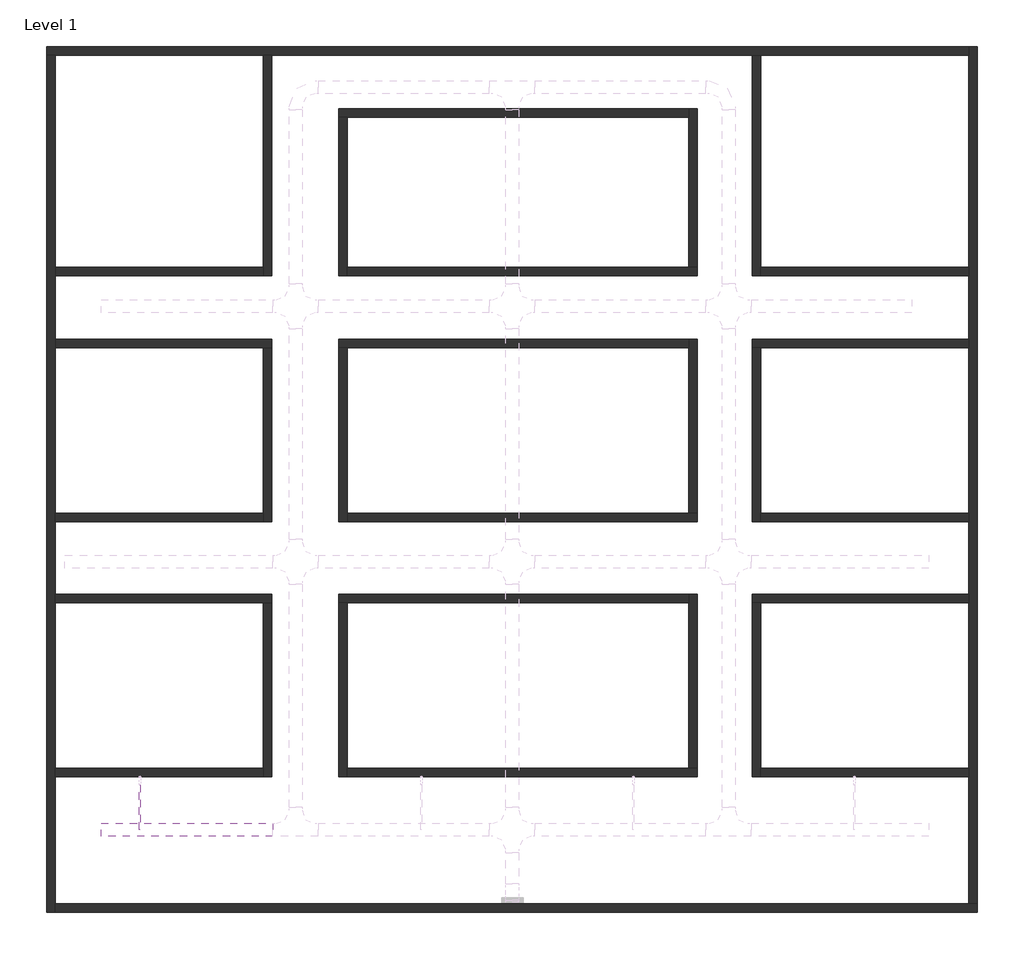
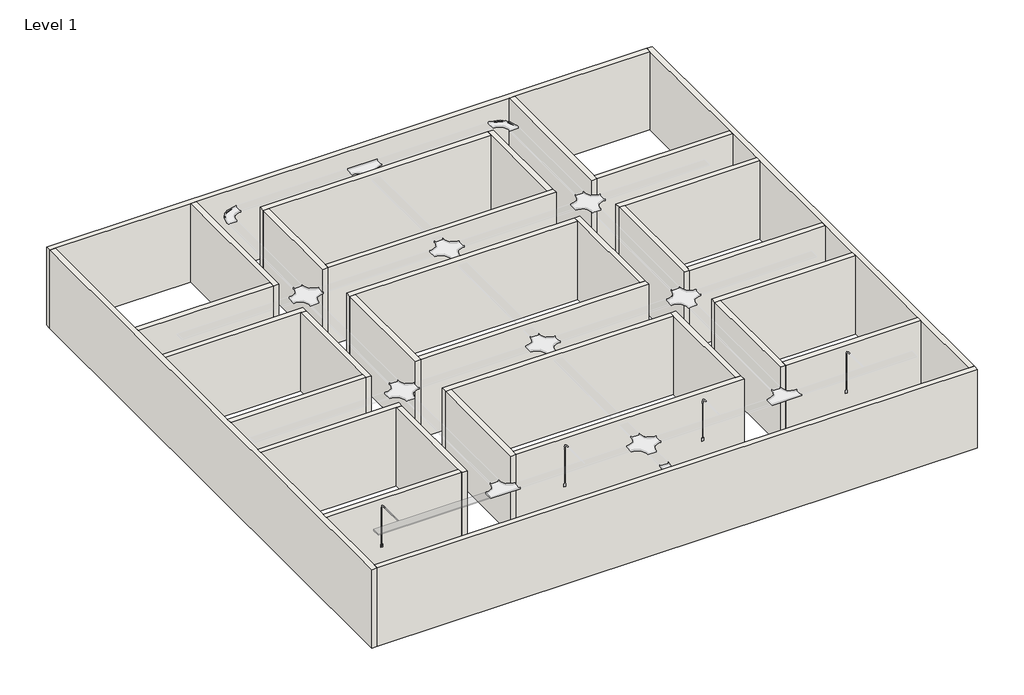
# One storey, part 1 of 2: 32 walls, 3 cable carrier segments, 1 proxy.
"""IFC4 building model written with IfcOpenShell, lengths in millimetres."""

import ifcopenshell
import ifcopenshell.guid

model = None  # the IFC model being written
_history = None  # IfcOwnerHistory: only IFC2X3 demands one
_inside = {}  # id of a spatial element -> (the spatial element, [elements in it])
_under = {}  # id of a project, library or spatial element -> (it, [spatial elements below it])
_declared = {}  # id of a project -> (the project, [libraries it declares])
_typed = {}  # id of a type object -> (the type object, [elements of that type])
_made_of = {}  # id of a material, layer set ... -> (it, [elements and type objects made of it])


def new_model(schema):
    """Start an empty IFC model of exactly this schema.

    Asked for "IFC4X3", IfcOpenShell would pick the latest addendum, in which some entities
    have other attributes; the version numbers below select the first issue.
    IFC2X3 requires an IfcOwnerHistory on every rooted entity: one is made here for all.
    """
    global model, _history
    if schema == "IFC4X3":
        model = ifcopenshell.file(schema_version=(4, 3, 0, 0))
    else:
        model = ifcopenshell.file(schema=schema)
    _inside.clear()
    _under.clear()
    _declared.clear()
    _typed.clear()
    _made_of.clear()
    _history = None
    if model.schema == "IFC2X3":
        org = make("IfcOrganization", Name="unknown")
        user = make(
            "IfcPersonAndOrganization",
            ThePerson=make("IfcPerson", FamilyName="unknown"),
            TheOrganization=org,
        )
        app = make(
            "IfcApplication",
            ApplicationDeveloper=org,
            Version="unknown",
            ApplicationFullName="unknown",
            ApplicationIdentifier="unknown",
        )
        _history = make(
            "IfcOwnerHistory",
            OwningUser=user,
            OwningApplication=app,
            ChangeAction="ADDED",
            CreationDate=0,
        )
    return model


def make(cls, **values):
    """One entity of the class cls with the attributes given. An attribute that is None is left unset."""
    return model.create_entity(
        cls, **{name: value for name, value in values.items() if value is not None}
    )


def rooted(cls, **values):
    """An entity with a GlobalId (a new one), such as an element, a storey or a relation."""
    return make(cls, GlobalId=ifcopenshell.guid.new(), OwnerHistory=_history, **values)


def si_unit(unit_type, name, prefix=None):
    """IfcSIUnit, for example si_unit("LENGTHUNIT", "METRE", prefix="MILLI")."""
    return make("IfcSIUnit", UnitType=unit_type, Prefix=prefix, Name=name)


def assignment(units):
    """IfcUnitAssignment: the units of a project."""
    return None if units is None else make("IfcUnitAssignment", Units=units)


def point(xyz):
    """IfcCartesianPoint."""
    return None if xyz is None else make("IfcCartesianPoint", Coordinates=xyz)


def direction(xyz):
    """IfcDirection."""
    return None if xyz is None else make("IfcDirection", DirectionRatios=xyz)


def frame(location, z_axis=None, x_axis=None):
    """IfcAxis2Placement3D, a coordinate frame: its origin and axes. An axis left out is left unset."""
    return make(
        "IfcAxis2Placement3D",
        Location=point(location),
        Axis=direction(z_axis),
        RefDirection=direction(x_axis),
    )


def frame_2d(location, x_axis=None):
    """IfcAxis2Placement2D, a coordinate frame in the plane: its origin and x axis."""
    return make(
        "IfcAxis2Placement2D", Location=point(location), RefDirection=direction(x_axis)
    )


def origin():
    """The frame at (0, 0, 0) with its axes left unset."""
    return frame((0.0, 0.0, 0.0))


def origin_with_axes():
    """The frame at (0, 0, 0) with the z axis (0, 0, 1) and the x axis (1, 0, 0) written out."""
    return frame((0.0, 0.0, 0.0), z_axis=(0.0, 0.0, 1.0), x_axis=(1.0, 0.0, 0.0))


def place(relative_to, where):
    """IfcLocalPlacement: puts the frame where relative to a parent placement (None: the world)."""
    return make(
        "IfcLocalPlacement", PlacementRelTo=relative_to, RelativePlacement=where
    )


def context(
    kind, dimensions, precision=None, world=None, true_north=None, identifier=None
):
    """IfcGeometricRepresentationContext, for example the 3D "Model" context."""
    return make(
        "IfcGeometricRepresentationContext",
        ContextIdentifier=identifier,
        ContextType=kind,
        CoordinateSpaceDimension=dimensions,
        Precision=precision,
        WorldCoordinateSystem=world,
        TrueNorth=true_north,
    )


def project(units=None, contexts=None):
    """IfcProject with its units and contexts."""
    return rooted(
        "IfcProject",
        Name="project",
        RepresentationContexts=contexts,
        UnitsInContext=assignment(units),
    )


def spatial(cls, under=None, at=None, **own):
    """A site, building, storey or space (cls), placed at a placement, below another one or the project."""
    s = rooted(cls, ObjectPlacement=at, **own)
    if under is not None:
        _under.setdefault(under.id(), (under, []))[1].append(s)
    return s


def polyline(points):
    """IfcPolyline through the points."""
    return make("IfcPolyline", Points=[point(p) for p in points])


def circle_curve(where, radius):
    """IfcCircle in the frame where."""
    return make("IfcCircle", Position=where, Radius=radius)


def trimmed(basis, trim1, trim2, sense, master):
    """IfcTrimmedCurve: the piece of a basis curve between two trims."""
    return make(
        "IfcTrimmedCurve",
        BasisCurve=basis,
        Trim1=trim1,
        Trim2=trim2,
        SenseAgreement=sense,
        MasterRepresentation=master,
    )


def segment(curve, same_sense, transition):
    """IfcCompositeCurveSegment."""
    return make(
        "IfcCompositeCurveSegment",
        Transition=transition,
        SameSense=same_sense,
        ParentCurve=curve,
    )


def composite_curve(segments, self_intersect=None):
    """IfcCompositeCurve: segments joined end to end."""
    return make("IfcCompositeCurve", Segments=segments, SelfIntersect=self_intersect)


def outline(outer, holes=None, kind="AREA"):
    """IfcArbitraryClosedProfileDef: a profile drawn as a closed curve; with holes, ...WithVoids."""
    if holes is None:
        return make("IfcArbitraryClosedProfileDef", ProfileType=kind, OuterCurve=outer)
    return make(
        "IfcArbitraryProfileDefWithVoids",
        ProfileType=kind,
        OuterCurve=outer,
        InnerCurves=holes,
    )


def extrude(swept, where, along, depth):
    """IfcExtrudedAreaSolid: the profile swept, set in the frame where, extruded along a direction by depth."""
    return make(
        "IfcExtrudedAreaSolid",
        SweptArea=swept,
        Position=where,
        ExtrudedDirection=direction(along),
        Depth=depth,
    )


def faces_of(points, faces, orient=None, outer=None):
    """IfcFace entities. A face is a list of loops; a loop is a list of indices into points, from 0.

    orient and outer hold one flag for each loop. By default every Orientation is true, the
    first loop of a face is its IfcFaceOuterBound and the others are IfcFaceBound.
    """
    made = []
    for i, loops in enumerate(faces):
        bounds = []
        for j, loop in enumerate(loops):
            is_outer = j == 0 if outer is None else outer[i][j]
            bounds.append(
                make(
                    "IfcFaceOuterBound" if is_outer else "IfcFaceBound",
                    Bound=make("IfcPolyLoop", Polygon=[points[k] for k in loop]),
                    Orientation=True if orient is None else orient[i][j],
                )
            )
        made.append(make("IfcFace", Bounds=bounds))
    return made


def faceted_brep(points, faces, orient=None, outer=None, voids=None):
    """IfcFacetedBrep: a solid bounded by flat faces; with voids (closed shells), ...WithVoids."""
    shared = [point(p) for p in points]
    hull = make("IfcClosedShell", CfsFaces=faces_of(shared, faces, orient, outer))
    if voids is None:
        return make("IfcFacetedBrep", Outer=hull)
    return make(
        "IfcFacetedBrepWithVoids",
        Outer=hull,
        Voids=[
            make(cls, CfsFaces=faces_of(shared, fs, o, b)) for cls, fs, o, b in voids
        ],
    )


def shape(context_of_items, identifier, shape_type, items):
    """IfcShapeRepresentation: the items that make up one representation, for example the "Body"."""
    return make(
        "IfcShapeRepresentation",
        ContextOfItems=context_of_items,
        RepresentationIdentifier=identifier,
        RepresentationType=shape_type,
        Items=items,
    )


def source(mapping_origin, context_of_items, identifier, shape_type, items):
    """IfcRepresentationMap: a shape defined once, which mapped items show again and again."""
    return make(
        "IfcRepresentationMap",
        MappingOrigin=mapping_origin,
        MappedRepresentation=shape(context_of_items, identifier, shape_type, items),
    )


def transform(
    local_origin,
    x_axis=None,
    y_axis=None,
    z_axis=None,
    scale=None,
    scale2=None,
    scale3=None,
    uniform=True,
):
    """IfcCartesianTransformationOperator3D, or its non-uniform kind. x_axis, y_axis, z_axis: its Axis1, 2, 3."""
    if uniform:
        return make(
            "IfcCartesianTransformationOperator3D",
            Axis1=direction(x_axis),
            Axis2=direction(y_axis),
            LocalOrigin=point(local_origin),
            Scale=scale,
            Axis3=direction(z_axis),
        )
    return make(
        "IfcCartesianTransformationOperator3DnonUniform",
        Axis1=direction(x_axis),
        Axis2=direction(y_axis),
        LocalOrigin=point(local_origin),
        Scale=scale,
        Axis3=direction(z_axis),
        Scale2=scale2,
        Scale3=scale3,
    )


def mapped(mapping_source, mapping_target):
    """IfcMappedItem: shows the shape of a source again, moved by a transform."""
    return make(
        "IfcMappedItem", MappingSource=mapping_source, MappingTarget=mapping_target
    )


def made_of(thing, what):
    """Note that an element or type object is made of a material, layer set ...; save() writes the relation."""
    if what is not None:
        _made_of.setdefault(what.id(), (what, []))[1].append(thing)
    return thing


def element(
    cls,
    number,
    at=None,
    inside=None,
    cuts=None,
    type_object=None,
    material=None,
    context=None,
    identifier="Body",
    shape_type=None,
    held_by="IfcProductDefinitionShape",
    body=None,
    shapes=None,
    **own,
):
    """One element of the class cls, such as IfcWall. Its Tag is "e" and its number.

    at: its placement. inside: the storey or other place that contains it. cuts: it is an
    opening in that element (IfcRelVoidsElement). A single representation is given by context,
    identifier, shape_type and body (its items); several are given by shapes. held_by: the class
    of the entity that holds the representations. save() writes the other relations.
    """
    e = rooted(cls, Tag="e%d" % number, ObjectPlacement=at, **own)
    if body is not None:
        shapes = [shape(context, identifier, shape_type, body)]
    if shapes is not None:
        e.Representation = make(held_by, Representations=shapes)
    if inside is not None:
        _inside.setdefault(inside.id(), (inside, []))[1].append(e)
    if cuts is not None:
        rooted(
            "IfcRelVoidsElement", RelatingBuildingElement=cuts, RelatedOpeningElement=e
        )
    if type_object is not None:
        _typed.setdefault(type_object.id(), (type_object, []))[1].append(e)
    return made_of(e, material)


def aggregate(whole, parts):
    """IfcRelAggregates: a whole, such as a stair, and the parts it consists of."""
    return rooted("IfcRelAggregates", RelatingObject=whole, RelatedObjects=parts)


def save(model, path):
    """Write the relations noted so far, then the file.

    IfcRelAggregates (storeys below a building ...), IfcRelContainedInSpatialStructure (elements
    in a storey), IfcRelDefinesByType, IfcRelAssociatesMaterial and IfcRelDeclares: one each for
    every whole, place, type object, material and project.
    """
    for whole, parts in _under.values():
        aggregate(whole, parts)
    for where, things in _inside.values():
        rooted(
            "IfcRelContainedInSpatialStructure",
            RelatedElements=things,
            RelatingStructure=where,
        )
    for kind, things in _typed.values():
        rooted("IfcRelDefinesByType", RelatedObjects=things, RelatingType=kind)
    for what, things in _made_of.values():
        rooted("IfcRelAssociatesMaterial", RelatedObjects=things, RelatingMaterial=what)
    for by, libraries in _declared.values():
        rooted("IfcRelDeclares", RelatingContext=by, RelatedDefinitions=libraries)
    model.write(path)


def duplex_receptacle_gfci_10251bba(model_context):
    return source(origin(), model_context, "Body", "SweptSolid", [
        extrude(outline(polyline([(19.05, 38.1), (19.05, -38.1), (-19.05, -38.1), (-19.05, 38.1), (19.05, 38.1)])), frame((0.0, 0.0, -53.975), z_axis=(0.0, 0.0, 1.0), x_axis=(1.0, 0.0, 0.0)), (0.0, 0.0, 1.0), 53.975),
        extrude(outline(polyline([(34.925, 57.15), (34.925, -57.15), (-34.925, -57.15), (-34.925, 57.15), (34.925, 57.15)])), origin_with_axes(), (0.0, 0.0, 1.0), 4.7625),
    ])


model = new_model("IFC4")

# Units and contexts
model_context = context("Model", 3, world=origin())
ifc_project = project(units=[si_unit("LENGTHUNIT", "METRE", prefix="MILLI")], contexts=[model_context])

# Site, building, storey
site = spatial("IfcSite", under=ifc_project)
building = spatial("IfcBuilding", under=site)
storey = spatial("IfcBuildingStorey", under=building, Name="Level 1", Elevation=0.0)

# Proxy
placement = place(None, origin())
duplex_receptacle_gfci_shape = duplex_receptacle_gfci_10251bba(model_context)
element("IfcBuildingElementProxy", 1, Name="Duplex Receptacle : GFCI", ObjectType="Duplex Receptacle : GFCI", at=placement, inside=storey, context=model_context, shape_type="MappedRepresentation", body=[
    mapped(duplex_receptacle_gfci_shape, transform((-9709.662063, -4539.6447766, 1219.2), x_axis=(1.0, 0.0, 0.0), y_axis=(0.0, 0.0, 1.0), z_axis=(0.0, -1.0, 0.0))),
])

# Cable carrier segments
element("IfcCableCarrierSegment", 2, ObjectType="Channel Cable Tray", at=placement, inside=storey, context=model_context, shape_type="SweptSolid", body=[
    extrude(outline(polyline([(-6575.0301128, -5642.9993215), (-6575.0301128, -5947.7993215), (-10619.5600084, -5947.7993215), (-10619.5600084, -5642.9993215), (-6575.0301128, -5642.9993215)])), frame((0.0, 0.0, 2774.6), z_axis=(0.0, 0.0, 1.0), x_axis=(1.0, 0.0, 0.0)), (0.0, 0.0, 1.0), 50.8),
])
element("IfcCableCarrierSegment", 3, ObjectType="Electrical Metallic Tubing (EMT)", at=placement, inside=storey, context=model_context, shape_type="SweptSolid", body=[
    extrude(outline(composite_curve([segment(trimmed(circle_curve(frame_2d((2800.0, -9709.662063)), 12.6999995), [point((2800.0, -9722.3620625))], [point((2787.3000005, -9709.662063))], False, "CARTESIAN"), True, "CONTINUOUS"), segment(trimmed(circle_curve(frame_2d((2800.0, -9709.662063)), 12.6999995), [point((2787.3000005, -9709.662063))], [point((2800.0, -9696.9620635))], False, "CARTESIAN"), True, "CONTINUOUS"), segment(trimmed(circle_curve(frame_2d((2800.0, -9709.662063)), 12.6999995), [point((2800.0, -9696.9620635))], [point((2812.6999995, -9709.662063))], False, "CARTESIAN"), True, "CONTINUOUS"), segment(trimmed(circle_curve(frame_2d((2800.0, -9709.662063)), 12.6999995), [point((2812.6999995, -9709.662063))], [point((2800.0, -9722.3620625))], False, "CARTESIAN"), True, "CONTINUOUS")], self_intersect=False)), frame((0.0, -5795.3993215, 0.0), z_axis=(0.0, 1.0, 0.0), x_axis=(0.0, 0.0, 1.0)), (0.0, 0.0, 1.0), 1062.17877),
])
element("IfcCableCarrierSegment", 4, ObjectType="Electrical Metallic Tubing (EMT)", at=placement, inside=storey, context=model_context, shape_type="SweptSolid", body=[
    extrude(outline(composite_curve([segment(trimmed(circle_curve(frame_2d((-9709.662063, -4539.6447766)), 12.6999995), [point((-9696.9620635, -4539.6447766))], [point((-9709.662063, -4552.3447761))], False, "CARTESIAN"), True, "CONTINUOUS"), segment(trimmed(circle_curve(frame_2d((-9709.662063, -4539.6447766)), 12.6999995), [point((-9709.662063, -4552.3447761))], [point((-9722.3620625, -4539.6447766))], False, "CARTESIAN"), True, "CONTINUOUS"), segment(trimmed(circle_curve(frame_2d((-9709.662063, -4539.6447766)), 12.6999995), [point((-9722.3620625, -4539.6447766))], [point((-9709.662063, -4526.9447771))], False, "CARTESIAN"), True, "CONTINUOUS"), segment(trimmed(circle_curve(frame_2d((-9709.662063, -4539.6447766)), 12.6999995), [point((-9709.662063, -4526.9447771))], [point((-9696.9620635, -4539.6447766))], False, "CARTESIAN"), True, "CONTINUOUS")], self_intersect=False)), frame((0.0, 0.0, 1219.2), z_axis=(0.0, 0.0, 1.0), x_axis=(1.0, 0.0, 0.0)), (0.0, 0.0, 1.0), 1387.2242251),
])

# Walls
element("IfcWall", 5, ObjectType="Generic - 200mm", at=placement, inside=storey, context=model_context, shape_type="Brep", body=[
    faceted_brep([(-11909.662063, 12460.3552234, 0.0), (-11709.662063, 12460.3552234, 0.0), (-6809.662063, 12460.3552234, 0.0), (-6609.662063, 12460.3552234, 0.0), (4722.664183, 12460.3552234, 0.0), (4922.664183, 12460.3552234, 0.0), (9822.664183, 12460.3552234, 0.0), (9822.664183, 12460.3552234, 3000.0), (4922.664183, 12460.3552234, 3000.0), (4722.664183, 12460.3552234, 3000.0), (-6609.662063, 12460.3552234, 3000.0), (-6809.662063, 12460.3552234, 3000.0), (-11709.662063, 12460.3552234, 3000.0), (-11909.662063, 12460.3552234, 3000.0), (-11909.662063, 12660.3552234, 0.0), (-11909.662063, 12660.3552234, 3000.0), (9822.664183, 12660.3552234, 3000.0), (9822.664183, 12660.3552234, 0.0)], [[[0, 1, 2, 3, 4, 5, 6, 7, 8, 9, 10, 11, 12, 13]], [[14, 15, 16, 17]], [[6, 5, 4, 3, 2, 1, 0, 14, 17]], [[13, 12, 11, 10, 9, 8, 7, 16, 15]], [[0, 13, 15, 14]], [[7, 6, 17, 16]]]),
])
element("IfcWall", 6, ObjectType="Generic - 200mm", at=placement, inside=storey, context=model_context, shape_type="Brep", body=[
    faceted_brep([(-11709.662063, -7739.6447766, 0.0), (-11709.662063, -7539.6447766, 0.0), (-11709.662063, -4539.6447766, 0.0), (-11709.662063, -4339.6447766, 0.0), (-11709.662063, -439.6447766, 0.0), (-11709.662063, -239.6447766, 0.0), (-11709.662063, 1460.3552234, 0.0), (-11709.662063, 1660.3552234, 0.0), (-11709.662063, 5560.3552234, 0.0), (-11709.662063, 5760.3552234, 0.0), (-11709.662063, 7260.3552234, 0.0), (-11709.662063, 7460.3552234, 0.0), (-11709.662063, 12460.3552234, 0.0), (-11709.662063, 12460.3552234, 3000.0), (-11709.662063, 7460.3552234, 3000.0), (-11709.662063, 7260.3552234, 3000.0), (-11709.662063, 5760.3552234, 3000.0), (-11709.662063, 5560.3552234, 3000.0), (-11709.662063, 1660.3552234, 3000.0), (-11709.662063, 1460.3552234, 3000.0), (-11709.662063, -239.6447766, 3000.0), (-11709.662063, -439.6447766, 3000.0), (-11709.662063, -4339.6447766, 3000.0), (-11709.662063, -4539.6447766, 3000.0), (-11709.662063, -7539.6447766, 3000.0), (-11709.662063, -7739.6447766, 3000.0), (-11909.662063, -7739.6447766, 0.0), (-11909.662063, -7739.6447766, 3000.0), (-11909.662063, 12460.3552234, 3000.0), (-11909.662063, 12460.3552234, 0.0)], [[[0, 1, 2, 3, 4, 5, 6, 7, 8, 9, 10, 11, 12, 13, 14, 15, 16, 17, 18, 19, 20, 21, 22, 23, 24, 25]], [[26, 27, 28, 29]], [[12, 11, 10, 9, 8, 7, 6, 5, 4, 3, 2, 1, 0, 26, 29]], [[25, 24, 23, 22, 21, 20, 19, 18, 17, 16, 15, 14, 13, 28, 27]], [[0, 25, 27, 26]], [[13, 12, 29, 28]]]),
])
element("IfcWall", 7, ObjectType="Generic - 200mm", at=placement, inside=storey, context=model_context, shape_type="Brep", body=[
    faceted_brep([(10022.664183, -7539.6447766, 0.0), (9822.664183, -7539.6447766, 0.0), (-11709.662063, -7539.6447766, 0.0), (-11709.662063, -7539.6447766, 3000.0), (9822.664183, -7539.6447766, 3000.0), (10022.664183, -7539.6447766, 3000.0), (10022.664183, -7739.6447766, 0.0), (10022.664183, -7739.6447766, 3000.0), (-11709.662063, -7739.6447766, 3000.0), (-11709.662063, -7739.6447766, 0.0)], [[[0, 1, 2, 3, 4, 5]], [[6, 7, 8, 9]], [[2, 1, 0, 6, 9]], [[5, 4, 3, 8, 7]], [[0, 5, 7, 6]], [[3, 2, 9, 8]]]),
])
element("IfcWall", 8, ObjectType="Generic - 200mm", at=placement, inside=storey, context=model_context, shape_type="Brep", body=[
    faceted_brep([(9822.664183, 12660.3552234, 0.0), (9822.664183, 12460.3552234, 0.0), (9822.664183, 7460.3552234, 0.0), (9822.664183, 7260.3552234, 0.0), (9822.664183, 5760.3552234, 0.0), (9822.664183, 5560.3552234, 0.0), (9822.664183, 1660.3552234, 0.0), (9822.664183, 1460.3552234, 0.0), (9822.664183, -239.6447766, 0.0), (9822.664183, -439.6447766, 0.0), (9822.664183, -4339.6447766, 0.0), (9822.664183, -4539.6447766, 0.0), (9822.664183, -7539.6447766, 0.0), (9822.664183, -7539.6447766, 3000.0), (9822.664183, -4539.6447766, 3000.0), (9822.664183, -4339.6447766, 3000.0), (9822.664183, -439.6447766, 3000.0), (9822.664183, -239.6447766, 3000.0), (9822.664183, 1460.3552234, 3000.0), (9822.664183, 1660.3552234, 3000.0), (9822.664183, 5560.3552234, 3000.0), (9822.664183, 5760.3552234, 3000.0), (9822.664183, 7260.3552234, 3000.0), (9822.664183, 7460.3552234, 3000.0), (9822.664183, 12460.3552234, 3000.0), (9822.664183, 12660.3552234, 3000.0), (10022.664183, 12660.3552234, 0.0), (10022.664183, 12660.3552234, 3000.0), (10022.664183, -7539.6447766, 3000.0), (10022.664183, -7539.6447766, 0.0)], [[[0, 1, 2, 3, 4, 5, 6, 7, 8, 9, 10, 11, 12, 13, 14, 15, 16, 17, 18, 19, 20, 21, 22, 23, 24, 25]], [[26, 27, 28, 29]], [[12, 11, 10, 9, 8, 7, 6, 5, 4, 3, 2, 1, 0, 26, 29]], [[25, 24, 23, 22, 21, 20, 19, 18, 17, 16, 15, 14, 13, 28, 27]], [[0, 25, 27, 26]], [[13, 12, 29, 28]]]),
])
element("IfcWall", 9, ObjectType="Generic - 200mm", at=placement, inside=storey, context=model_context, shape_type="Brep", body=[
    faceted_brep([(-6809.662063, -439.6447766, 0.0), (-6809.662063, -4339.6447766, 0.0), (-6809.662063, -4539.6447766, 0.0), (-6809.662063, -4539.6447766, 3000.0), (-6809.662063, -4339.6447766, 3000.0), (-6809.662063, -439.6447766, 3000.0), (-6609.662063, -439.6447766, 0.0), (-6609.662063, -439.6447766, 3000.0), (-6609.662063, -4539.6447766, 3000.0), (-6609.662063, -4539.6447766, 0.0)], [[[0, 1, 2, 3, 4, 5]], [[6, 7, 8, 9]], [[2, 1, 0, 6, 9]], [[5, 4, 3, 8, 7]], [[3, 2, 9, 8]], [[0, 5, 7, 6]]]),
])
element("IfcWall", 10, ObjectType="Generic - 200mm", at=placement, inside=storey, context=model_context, shape_type="SweptSolid", body=[
    extrude(outline(polyline([(-11709.662063, -4339.6447766), (-6809.662063, -4339.6447766), (-6809.662063, -4539.6447766), (-11709.662063, -4539.6447766), (-11709.662063, -4339.6447766)])), origin_with_axes(), (0.0, 0.0, 1.0), 3000.0),
])
element("IfcWall", 11, ObjectType="Generic - 200mm", at=placement, inside=storey, context=model_context, shape_type="Brep", body=[
    faceted_brep([(-11709.662063, -439.6447766, 0.0), (-6809.662063, -439.6447766, 0.0), (-6609.662063, -439.6447766, 0.0), (-6609.662063, -439.6447766, 3000.0), (-6809.662063, -439.6447766, 3000.0), (-11709.662063, -439.6447766, 3000.0), (-11709.662063, -239.6447766, 0.0), (-11709.662063, -239.6447766, 3000.0), (-6609.662063, -239.6447766, 3000.0), (-6609.662063, -239.6447766, 0.0)], [[[0, 1, 2, 3, 4, 5]], [[6, 7, 8, 9]], [[2, 1, 0, 6, 9]], [[5, 4, 3, 8, 7]], [[0, 5, 7, 6]], [[3, 2, 9, 8]]]),
])
element("IfcWall", 12, ObjectType="Generic - 200mm", at=placement, inside=storey, context=model_context, shape_type="Brep", body=[
    faceted_brep([(-6809.662063, 5560.3552234, 0.0), (-6809.662063, 1660.3552234, 0.0), (-6809.662063, 1460.3552234, 0.0), (-6809.662063, 1460.3552234, 3000.0), (-6809.662063, 1660.3552234, 3000.0), (-6809.662063, 5560.3552234, 3000.0), (-6609.662063, 5560.3552234, 0.0), (-6609.662063, 5560.3552234, 3000.0), (-6609.662063, 1460.3552234, 3000.0), (-6609.662063, 1460.3552234, 0.0)], [[[0, 1, 2, 3, 4, 5]], [[6, 7, 8, 9]], [[2, 1, 0, 6, 9]], [[5, 4, 3, 8, 7]], [[3, 2, 9, 8]], [[0, 5, 7, 6]]]),
])
element("IfcWall", 13, ObjectType="Generic - 200mm", at=placement, inside=storey, context=model_context, shape_type="SweptSolid", body=[
    extrude(outline(polyline([(-11709.662063, 1660.3552234), (-6809.662063, 1660.3552234), (-6809.662063, 1460.3552234), (-11709.662063, 1460.3552234), (-11709.662063, 1660.3552234)])), origin_with_axes(), (0.0, 0.0, 1.0), 3000.0),
])
element("IfcWall", 14, ObjectType="Generic - 200mm", at=placement, inside=storey, context=model_context, shape_type="Brep", body=[
    faceted_brep([(-11709.662063, 5560.3552234, 0.0), (-6809.662063, 5560.3552234, 0.0), (-6609.662063, 5560.3552234, 0.0), (-6609.662063, 5560.3552234, 3000.0), (-6809.662063, 5560.3552234, 3000.0), (-11709.662063, 5560.3552234, 3000.0), (-11709.662063, 5760.3552234, 0.0), (-11709.662063, 5760.3552234, 3000.0), (-6609.662063, 5760.3552234, 3000.0), (-6609.662063, 5760.3552234, 0.0)], [[[0, 1, 2, 3, 4, 5]], [[6, 7, 8, 9]], [[2, 1, 0, 6, 9]], [[5, 4, 3, 8, 7]], [[3, 2, 9, 8]], [[0, 5, 7, 6]]]),
])
element("IfcWall", 15, ObjectType="Generic - 200mm", at=placement, inside=storey, context=model_context, shape_type="Brep", body=[
    faceted_brep([(-6809.662063, 12460.3552234, 0.0), (-6809.662063, 7460.3552234, 0.0), (-6809.662063, 7260.3552234, 0.0), (-6809.662063, 7260.3552234, 3000.0), (-6809.662063, 7460.3552234, 3000.0), (-6809.662063, 12460.3552234, 3000.0), (-6609.662063, 12460.3552234, 0.0), (-6609.662063, 12460.3552234, 3000.0), (-6609.662063, 7260.3552234, 3000.0), (-6609.662063, 7260.3552234, 0.0)], [[[0, 1, 2, 3, 4, 5]], [[6, 7, 8, 9]], [[2, 1, 0, 6, 9]], [[5, 4, 3, 8, 7]], [[3, 2, 9, 8]], [[0, 5, 7, 6]]]),
])
element("IfcWall", 16, ObjectType="Generic - 200mm", at=placement, inside=storey, context=model_context, shape_type="SweptSolid", body=[
    extrude(outline(polyline([(-11709.662063, 7460.3552234), (-6809.662063, 7460.3552234), (-6809.662063, 7260.3552234), (-11709.662063, 7260.3552234), (-11709.662063, 7460.3552234)])), origin_with_axes(), (0.0, 0.0, 1.0), 3000.0),
])
element("IfcWall", 17, ObjectType="Generic - 200mm", at=placement, inside=storey, context=model_context, shape_type="Brep", body=[
    faceted_brep([(-5023.4293583, 10991.3898121, 0.0), (-4823.4293583, 10991.3898121, 0.0), (3222.664183, 10991.3898121, 0.0), (3222.664183, 10991.3898121, 3000.0), (-4823.4293583, 10991.3898121, 3000.0), (-5023.4293583, 10991.3898121, 3000.0), (-5023.4293583, 11191.3898121, 0.0), (-5023.4293583, 11191.3898121, 3000.0), (3222.664183, 11191.3898121, 3000.0), (3222.664183, 11191.3898121, 0.0)], [[[0, 1, 2, 3, 4, 5]], [[6, 7, 8, 9]], [[2, 1, 0, 6, 9]], [[5, 4, 3, 8, 7]], [[0, 5, 7, 6]], [[3, 2, 9, 8]]]),
])
element("IfcWall", 18, ObjectType="Generic - 200mm", at=placement, inside=storey, context=model_context, shape_type="Brep", body=[
    faceted_brep([(-4823.4293583, 7260.3552234, 0.0), (-4823.4293583, 7460.3552234, 0.0), (-4823.4293583, 10991.3898121, 0.0), (-4823.4293583, 10991.3898121, 3000.0), (-4823.4293583, 7460.3552234, 3000.0), (-4823.4293583, 7260.3552234, 3000.0), (-5023.4293583, 7260.3552234, 0.0), (-5023.4293583, 7260.3552234, 3000.0), (-5023.4293583, 10991.3898121, 3000.0), (-5023.4293583, 10991.3898121, 0.0)], [[[0, 1, 2, 3, 4, 5]], [[6, 7, 8, 9]], [[2, 1, 0, 6, 9]], [[5, 4, 3, 8, 7]], [[0, 5, 7, 6]], [[3, 2, 9, 8]]]),
])
element("IfcWall", 19, ObjectType="Generic - 200mm", at=placement, inside=storey, context=model_context, shape_type="Brep", body=[
    faceted_brep([(3422.664183, 7460.3552234, 0.0), (3222.664183, 7460.3552234, 0.0), (-4823.4293583, 7460.3552234, 0.0), (-4823.4293583, 7460.3552234, 3000.0), (3222.664183, 7460.3552234, 3000.0), (3422.664183, 7460.3552234, 3000.0), (3422.664183, 7260.3552234, 0.0), (3422.664183, 7260.3552234, 3000.0), (-4823.4293583, 7260.3552234, 3000.0), (-4823.4293583, 7260.3552234, 0.0)], [[[0, 1, 2, 3, 4, 5]], [[6, 7, 8, 9]], [[2, 1, 0, 6, 9]], [[5, 4, 3, 8, 7]], [[0, 5, 7, 6]], [[3, 2, 9, 8]]]),
])
element("IfcWall", 20, ObjectType="Generic - 200mm", at=placement, inside=storey, context=model_context, shape_type="Brep", body=[
    faceted_brep([(3222.664183, 11191.3898121, 0.0), (3222.664183, 10991.3898121, 0.0), (3222.664183, 7460.3552234, 0.0), (3222.664183, 7460.3552234, 3000.0), (3222.664183, 10991.3898121, 3000.0), (3222.664183, 11191.3898121, 3000.0), (3422.664183, 11191.3898121, 0.0), (3422.664183, 11191.3898121, 3000.0), (3422.664183, 7460.3552234, 3000.0), (3422.664183, 7460.3552234, 0.0)], [[[0, 1, 2, 3, 4, 5]], [[6, 7, 8, 9]], [[2, 1, 0, 6, 9]], [[5, 4, 3, 8, 7]], [[0, 5, 7, 6]], [[3, 2, 9, 8]]]),
])
element("IfcWall", 21, ObjectType="Generic - 200mm", at=placement, inside=storey, context=model_context, shape_type="Brep", body=[
    faceted_brep([(-5023.4293583, 5560.3552234, 0.0), (-4823.4293583, 5560.3552234, 0.0), (3222.664183, 5560.3552234, 0.0), (3222.664183, 5560.3552234, 3000.0), (-4823.4293583, 5560.3552234, 3000.0), (-5023.4293583, 5560.3552234, 3000.0), (-5023.4293583, 5760.3552234, 0.0), (-5023.4293583, 5760.3552234, 3000.0), (3222.664183, 5760.3552234, 3000.0), (3222.664183, 5760.3552234, 0.0)], [[[0, 1, 2, 3, 4, 5]], [[6, 7, 8, 9]], [[2, 1, 0, 6, 9]], [[5, 4, 3, 8, 7]], [[0, 5, 7, 6]], [[3, 2, 9, 8]]]),
])
element("IfcWall", 22, ObjectType="Generic - 200mm", at=placement, inside=storey, context=model_context, shape_type="Brep", body=[
    faceted_brep([(-4823.4293583, 1460.3552234, 0.0), (-4823.4293583, 1660.3552234, 0.0), (-4823.4293583, 5560.3552234, 0.0), (-4823.4293583, 5560.3552234, 3000.0), (-4823.4293583, 1660.3552234, 3000.0), (-4823.4293583, 1460.3552234, 3000.0), (-5023.4293583, 1460.3552234, 0.0), (-5023.4293583, 1460.3552234, 3000.0), (-5023.4293583, 5560.3552234, 3000.0), (-5023.4293583, 5560.3552234, 0.0)], [[[0, 1, 2, 3, 4, 5]], [[6, 7, 8, 9]], [[2, 1, 0, 6, 9]], [[5, 4, 3, 8, 7]], [[0, 5, 7, 6]], [[3, 2, 9, 8]]]),
])
element("IfcWall", 23, ObjectType="Generic - 200mm", at=placement, inside=storey, context=model_context, shape_type="Brep", body=[
    faceted_brep([(3422.664183, 1660.3552234, 0.0), (3222.664183, 1660.3552234, 0.0), (-4823.4293583, 1660.3552234, 0.0), (-4823.4293583, 1660.3552234, 3000.0), (3222.664183, 1660.3552234, 3000.0), (3422.664183, 1660.3552234, 3000.0), (3422.664183, 1460.3552234, 0.0), (3422.664183, 1460.3552234, 3000.0), (-4823.4293583, 1460.3552234, 3000.0), (-4823.4293583, 1460.3552234, 0.0)], [[[0, 1, 2, 3, 4, 5]], [[6, 7, 8, 9]], [[2, 1, 0, 6, 9]], [[5, 4, 3, 8, 7]], [[0, 5, 7, 6]], [[3, 2, 9, 8]]]),
])
element("IfcWall", 24, ObjectType="Generic - 200mm", at=placement, inside=storey, context=model_context, shape_type="Brep", body=[
    faceted_brep([(3222.664183, 5760.3552234, 0.0), (3222.664183, 5560.3552234, 0.0), (3222.664183, 1660.3552234, 0.0), (3222.664183, 1660.3552234, 3000.0), (3222.664183, 5560.3552234, 3000.0), (3222.664183, 5760.3552234, 3000.0), (3422.664183, 5760.3552234, 0.0), (3422.664183, 5760.3552234, 3000.0), (3422.664183, 1660.3552234, 3000.0), (3422.664183, 1660.3552234, 0.0)], [[[0, 1, 2, 3, 4, 5]], [[6, 7, 8, 9]], [[2, 1, 0, 6, 9]], [[5, 4, 3, 8, 7]], [[0, 5, 7, 6]], [[3, 2, 9, 8]]]),
])
element("IfcWall", 25, ObjectType="Generic - 200mm", at=placement, inside=storey, context=model_context, shape_type="Brep", body=[
    faceted_brep([(-5023.4293583, -439.6447766, 0.0), (-4823.4293583, -439.6447766, 0.0), (3222.664183, -439.6447766, 0.0), (3222.664183, -439.6447766, 3000.0), (-4823.4293583, -439.6447766, 3000.0), (-5023.4293583, -439.6447766, 3000.0), (-5023.4293583, -239.6447766, 0.0), (-5023.4293583, -239.6447766, 3000.0), (3222.664183, -239.6447766, 3000.0), (3222.664183, -239.6447766, 0.0)], [[[0, 1, 2, 3, 4, 5]], [[6, 7, 8, 9]], [[2, 1, 0, 6, 9]], [[5, 4, 3, 8, 7]], [[0, 5, 7, 6]], [[3, 2, 9, 8]]]),
])
element("IfcWall", 26, ObjectType="Generic - 200mm", at=placement, inside=storey, context=model_context, shape_type="Brep", body=[
    faceted_brep([(-4823.4293583, -4539.6447766, 0.0), (-4823.4293583, -4339.6447766, 0.0), (-4823.4293583, -439.6447766, 0.0), (-4823.4293583, -439.6447766, 3000.0), (-4823.4293583, -4339.6447766, 3000.0), (-4823.4293583, -4539.6447766, 3000.0), (-5023.4293583, -4539.6447766, 0.0), (-5023.4293583, -4539.6447766, 3000.0), (-5023.4293583, -439.6447766, 3000.0), (-5023.4293583, -439.6447766, 0.0)], [[[0, 1, 2, 3, 4, 5]], [[6, 7, 8, 9]], [[2, 1, 0, 6, 9]], [[5, 4, 3, 8, 7]], [[0, 5, 7, 6]], [[3, 2, 9, 8]]]),
])
element("IfcWall", 27, ObjectType="Generic - 200mm", at=placement, inside=storey, context=model_context, shape_type="Brep", body=[
    faceted_brep([(3422.664183, -4339.6447766, 0.0), (3222.664183, -4339.6447766, 0.0), (-4823.4293583, -4339.6447766, 0.0), (-4823.4293583, -4339.6447766, 3000.0), (3222.664183, -4339.6447766, 3000.0), (3422.664183, -4339.6447766, 3000.0), (3422.664183, -4539.6447766, 0.0), (3422.664183, -4539.6447766, 3000.0), (-4823.4293583, -4539.6447766, 3000.0), (-4823.4293583, -4539.6447766, 0.0)], [[[0, 1, 2, 3, 4, 5]], [[6, 7, 8, 9]], [[2, 1, 0, 6, 9]], [[5, 4, 3, 8, 7]], [[0, 5, 7, 6]], [[3, 2, 9, 8]]]),
])
element("IfcWall", 28, ObjectType="Generic - 200mm", at=placement, inside=storey, context=model_context, shape_type="Brep", body=[
    faceted_brep([(3222.664183, -239.6447766, 0.0), (3222.664183, -439.6447766, 0.0), (3222.664183, -4339.6447766, 0.0), (3222.664183, -4339.6447766, 3000.0), (3222.664183, -439.6447766, 3000.0), (3222.664183, -239.6447766, 3000.0), (3422.664183, -239.6447766, 0.0), (3422.664183, -239.6447766, 3000.0), (3422.664183, -4339.6447766, 3000.0), (3422.664183, -4339.6447766, 0.0)], [[[0, 1, 2, 3, 4, 5]], [[6, 7, 8, 9]], [[2, 1, 0, 6, 9]], [[5, 4, 3, 8, 7]], [[0, 5, 7, 6]], [[3, 2, 9, 8]]]),
])
element("IfcWall", 29, ObjectType="Generic - 200mm", at=placement, inside=storey, context=model_context, shape_type="Brep", body=[
    faceted_brep([(4722.664183, -439.6447766, 0.0), (4722.664183, -4539.6447766, 0.0), (4722.664183, -4539.6447766, 3000.0), (4722.664183, -439.6447766, 3000.0), (4922.664183, -439.6447766, 0.0), (4922.664183, -439.6447766, 3000.0), (4922.664183, -4339.6447766, 3000.0), (4922.664183, -4539.6447766, 3000.0), (4922.664183, -4539.6447766, 0.0), (4922.664183, -4339.6447766, 0.0)], [[[0, 1, 2, 3]], [[4, 5, 6, 7, 8, 9]], [[1, 0, 4, 9, 8]], [[3, 2, 7, 6, 5]], [[2, 1, 8, 7]], [[0, 3, 5, 4]]]),
])
element("IfcWall", 30, ObjectType="Generic - 200mm", at=placement, inside=storey, context=model_context, shape_type="SweptSolid", body=[
    extrude(outline(polyline([(9822.664183, -4539.6447766), (4922.664183, -4539.6447766), (4922.664183, -4339.6447766), (9822.664183, -4339.6447766), (9822.664183, -4539.6447766)])), origin_with_axes(), (0.0, 0.0, 1.0), 3000.0),
])
element("IfcWall", 31, ObjectType="Generic - 200mm", at=placement, inside=storey, context=model_context, shape_type="Brep", body=[
    faceted_brep([(9822.664183, -239.6447766, 0.0), (4722.664183, -239.6447766, 0.0), (4722.664183, -239.6447766, 3000.0), (9822.664183, -239.6447766, 3000.0), (9822.664183, -439.6447766, 0.0), (9822.664183, -439.6447766, 3000.0), (4922.664183, -439.6447766, 3000.0), (4722.664183, -439.6447766, 3000.0), (4722.664183, -439.6447766, 0.0), (4922.664183, -439.6447766, 0.0)], [[[0, 1, 2, 3]], [[4, 5, 6, 7, 8, 9]], [[1, 0, 4, 9, 8]], [[3, 2, 7, 6, 5]], [[2, 1, 8, 7]], [[0, 3, 5, 4]]]),
])
element("IfcWall", 32, ObjectType="Generic - 200mm", at=placement, inside=storey, context=model_context, shape_type="Brep", body=[
    faceted_brep([(4722.664183, 5560.3552234, 0.0), (4722.664183, 1460.3552234, 0.0), (4722.664183, 1460.3552234, 3000.0), (4722.664183, 5560.3552234, 3000.0), (4922.664183, 5560.3552234, 0.0), (4922.664183, 5560.3552234, 3000.0), (4922.664183, 1660.3552234, 3000.0), (4922.664183, 1460.3552234, 3000.0), (4922.664183, 1460.3552234, 0.0), (4922.664183, 1660.3552234, 0.0)], [[[0, 1, 2, 3]], [[4, 5, 6, 7, 8, 9]], [[1, 0, 4, 9, 8]], [[3, 2, 7, 6, 5]], [[2, 1, 8, 7]], [[0, 3, 5, 4]]]),
])
element("IfcWall", 33, ObjectType="Generic - 200mm", at=placement, inside=storey, context=model_context, shape_type="SweptSolid", body=[
    extrude(outline(polyline([(9822.664183, 1460.3552234), (4922.664183, 1460.3552234), (4922.664183, 1660.3552234), (9822.664183, 1660.3552234), (9822.664183, 1460.3552234)])), origin_with_axes(), (0.0, 0.0, 1.0), 3000.0),
])
element("IfcWall", 34, ObjectType="Generic - 200mm", at=placement, inside=storey, context=model_context, shape_type="Brep", body=[
    faceted_brep([(9822.664183, 5760.3552234, 0.0), (4722.664183, 5760.3552234, 0.0), (4722.664183, 5760.3552234, 3000.0), (9822.664183, 5760.3552234, 3000.0), (9822.664183, 5560.3552234, 0.0), (9822.664183, 5560.3552234, 3000.0), (4922.664183, 5560.3552234, 3000.0), (4722.664183, 5560.3552234, 3000.0), (4722.664183, 5560.3552234, 0.0), (4922.664183, 5560.3552234, 0.0)], [[[0, 1, 2, 3]], [[4, 5, 6, 7, 8, 9]], [[1, 0, 4, 9, 8]], [[3, 2, 7, 6, 5]], [[2, 1, 8, 7]], [[0, 3, 5, 4]]]),
])
element("IfcWall", 35, ObjectType="Generic - 200mm", at=placement, inside=storey, context=model_context, shape_type="Brep", body=[
    faceted_brep([(4722.664183, 12460.3552234, 0.0), (4722.664183, 7260.3552234, 0.0), (4722.664183, 7260.3552234, 3000.0), (4722.664183, 12460.3552234, 3000.0), (4922.664183, 12460.3552234, 0.0), (4922.664183, 12460.3552234, 3000.0), (4922.664183, 7460.3552234, 3000.0), (4922.664183, 7260.3552234, 3000.0), (4922.664183, 7260.3552234, 0.0), (4922.664183, 7460.3552234, 0.0)], [[[0, 1, 2, 3]], [[4, 5, 6, 7, 8, 9]], [[1, 0, 4, 9, 8]], [[3, 2, 7, 6, 5]], [[2, 1, 8, 7]], [[0, 3, 5, 4]]]),
])
element("IfcWall", 36, ObjectType="Generic - 200mm", at=placement, inside=storey, context=model_context, shape_type="SweptSolid", body=[
    extrude(outline(polyline([(9822.664183, 7260.3552234), (4922.664183, 7260.3552234), (4922.664183, 7460.3552234), (9822.664183, 7460.3552234), (9822.664183, 7260.3552234)])), origin_with_axes(), (0.0, 0.0, 1.0), 3000.0),
])

save(model, "model.ifc")

# Revit data of these elements
# Project information
#   Project Issue Date = "Issue Date"
#   Project Status = "Project Status"
#   Client Name = "Owner"
#   Project Address = "Enter address here"
#   Project Name = "Project Name"
#   Project Number = "Project Number"
# Type "Duplex Receptacle : GFCI"
#   Label = "GFCI"
#   Switch Voltage = 120 V
#   Load = 180 VA
#   Default Elevation = 1.2192 m
#   Load Classification = Receptacle
#   Assembly Code = ""
# Type "Generic - 200mm"
#   Layers, outside or top first: 0.2 m no material (function 1)
# Element 1 (IfcBuildingElementProxy, "Duplex Receptacle : GFCI")
#   Mark = "15"
#   Phase Created = New Construction
# Element 2 (IfcCableCarrierSegment, "Channel Cable Tray")
#   Phase Created = New Construction
#   section width or diameter = 0.3048 m
#   section height = 0.0508 m
# Elements 3, 4 (IfcCableCarrierSegment, "Electrical Metallic Tubing (EMT)")
#   Comments = ""
#   Phase Created = New Construction
#   section width or diameter = 0.0254 m
#   section height = 0.0254 m
# Elements 5, 6, 7, 8, 9, 10, 11, 12, 13, 14, 15, 16, 17, 18, 19, 20, 21, 22, 23, 24, 25, 26, 27, 28, 29, 30, 31, 32, 33, 34, 35, 36 (IfcWall, "Generic - 200mm")
#   Top Offset = 0 m
#   Base Offset = 0 m
#   Unconnected Height = 3 m
#   wall height = 3 m
#   Phase Created = New Construction
#   Base Constraint = Level 1
#   Materials on its faces: "Default Wall"
# Materials
#   "Default Wall": class "Miscellaneous", colour RGB 128 128 128, transparency 0, Cost = 0
